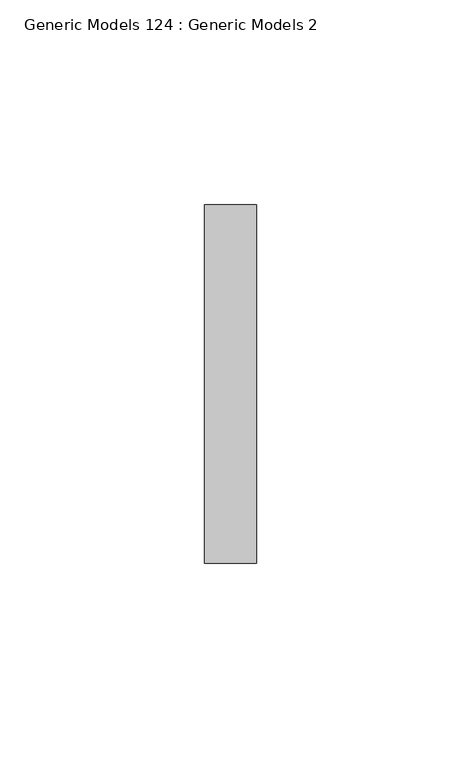
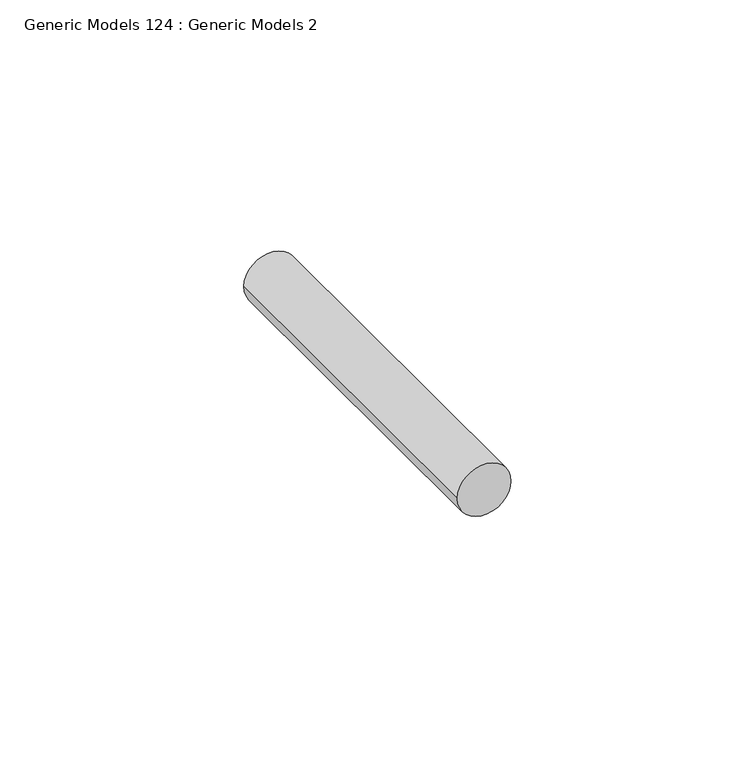
"""IFC4 building model written with IfcOpenShell, lengths in millimetres: proxy geometry, Generic Models 124 : Generic Models 2."""

from ifc_helpers import new_model, si_unit, point, frame, frame_2d, origin, place, context, project, spatial, circle_curve, trimmed, segment, composite_curve, outline, extrude, source, transform, mapped, element, save


def generic_models_124_generic_models_2_d576dfd6(model_context):
    return source(origin(), model_context, "Body", "SweptSolid", [
        extrude(outline(composite_curve([segment(trimmed(circle_curve(frame_2d((38203.4419837, 7297.5346014)), 6.35), [point((38203.4419837, 7303.8846014))], [point((38203.4419837, 7291.1846014))], False, "CARTESIAN"), True, "CONTINUOUS"), segment(trimmed(circle_curve(frame_2d((38203.4419837, 7297.5346014)), 6.35), [point((38203.4419837, 7291.1846014))], [point((38203.4419837, 7303.8846014))], False, "CARTESIAN"), True, "CONTINUOUS")], self_intersect=False)), frame((0.0, 1848.3666731, 0.0), z_axis=(0.0, 1.0, 0.0), x_axis=(0.0, 0.0, 1.0)), (0.0, 0.0, 1.0), 87.551022),
    ])


if __name__ == "__main__":
    model = new_model("IFC4")
    model_context = context("Model", 3, world=origin())
    ifc_project = project(units=[si_unit("LENGTHUNIT", "METRE", prefix="MILLI")], contexts=[model_context])
    site = spatial("IfcSite", under=ifc_project)
    building = spatial("IfcBuilding", under=site)
    placement = place(None, origin())
    generic_models_124_generic_models_2_shape = generic_models_124_generic_models_2_d576dfd6(model_context)
    element("IfcBuildingElementProxy", 1, Name="Generic Models 124 : Generic Models 2", ObjectType="Generic Models 124 : Generic Models 2", at=placement, inside=building, context=model_context, shape_type="MappedRepresentation", body=[
        mapped(generic_models_124_generic_models_2_shape, transform((0.0, 0.0, 0.0), x_axis=(1.0, 0.0, 0.0), y_axis=(0.0, 1.0, 0.0), z_axis=(0.0, 0.0, 1.0))),
    ])
    save(model, "model.ifc")

# Revit data of these elements
# Element 1 (IfcBuildingElementProxy, "Generic Models 124 : Generic Models 2")
#   Materials on its faces: "S.S. LAG BOLT - SEE STRUCT. DWGS"
# Materials
#   "S.S. LAG BOLT - SEE STRUCT. DWGS": class "Generic", colour RGB 120 120 120, transparency 0, Cost = 0
